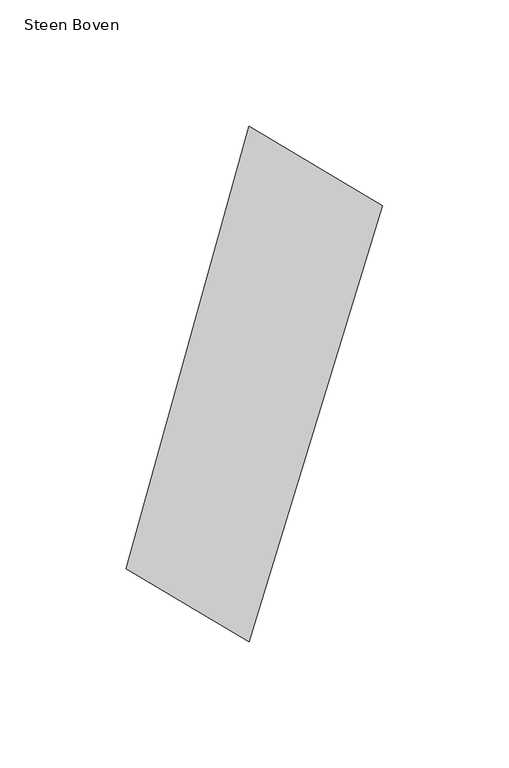
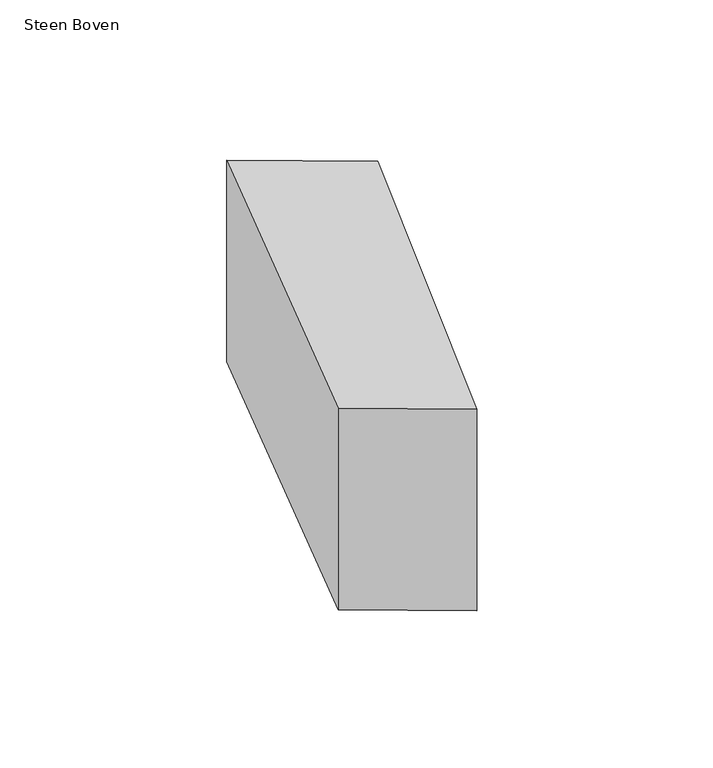
"""IFC4 building model written with IfcOpenShell, lengths in millimetres: proxy geometry, 00_GMA_steen_versie_4 : Steen Boven."""

from ifc_helpers import new_model, si_unit, origin, origin_with_axes, place, context, project, spatial, polyline, outline, extrude, source, transform, mapped, element, save


def steen_boven_836297aa(model_context):
    return source(origin(), model_context, "Body", "SweptSolid", [
        extrude(outline(polyline([(128.4213736, 159.6915758), (75.5524406, -12.6144697), (27.032959, 16.1703756), (75.6062, 191.0607778), (128.4213736, 159.6915758)])), origin_with_axes(), (0.0, 0.0, 1.0), 100.0),
    ])


if __name__ == "__main__":
    model = new_model("IFC4")
    model_context = context("Model", 3, world=origin())
    ifc_project = project(units=[si_unit("LENGTHUNIT", "METRE", prefix="MILLI")], contexts=[model_context])
    site = spatial("IfcSite", under=ifc_project)
    building = spatial("IfcBuilding", under=site)
    placement = place(None, origin())
    steen_boven_shape = steen_boven_836297aa(model_context)
    element("IfcBuildingElementProxy", 1, Name="00_GMA_steen_versie_4 : Steen Boven", ObjectType="00_GMA_steen_versie_4 : Steen Boven", at=placement, inside=building, context=model_context, shape_type="MappedRepresentation", body=[
        mapped(steen_boven_shape, transform((0.0, 0.0, 0.0), x_axis=(1.0, 0.0, 0.0), y_axis=(0.0, 1.0, 0.0), z_axis=(0.0, 0.0, 1.0))),
    ])
    save(model, "model.ifc")

# Revit data of these elements
# Type "00_GMA_steen_versie_4 : Steen Boven"
#   StootVoegHalfBoven [instance default] = 5 mm
#   StootVoegHalf [instance default] = 5 mm
#   StootVoegBreedteOnder = 10 mm
#   StootVoegBreedteBoven = 10 mm
#   Steendikte = 100 mm
#   LintVoegOnderHalf = 5 mm
#   LintVoegOnder = 10 mm
#   LintVoegBovenHalf = 0 mm
#   LintVoegBoven = 0 mm
#   materiaal = none
#   MateriaalVoeg = none
#   Default Elevation = 0
